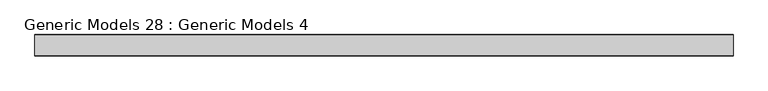
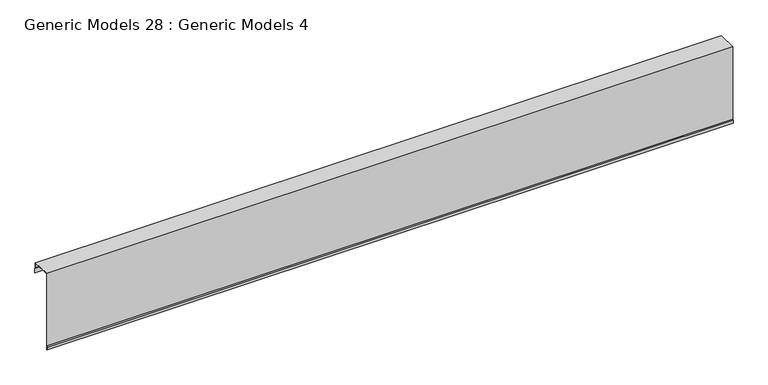
"""IFC4 building model written with IfcOpenShell, lengths in millimetres: proxy geometry, Generic Models 28 : Generic Models 4."""

from ifc_helpers import new_model, si_unit, frame, origin, place, context, project, spatial, polyline, outline, extrude, source, transform, mapped, element, save


def generic_models_28_generic_models_4_6f23a58d(model_context):
    return source(origin(), model_context, "Body", "SweptSolid", [
        extrude(outline(polyline([(-6892.3785185, 127021.0124798), (-6894.9743325, 127028.1444203), (-6894.9743325, 127077.8147702), (-7077.6823532, 127085.4276044), (-7077.6823532, 126394.6532716), (-7079.9703208, 126384.7429952), (-7079.9703208, 126359.7294973), (-7080.7640708, 126359.7294973), (-7080.7640708, 126384.8334316), (-7078.4761032, 126394.743708), (-7078.4761032, 127086.255116), (-6894.1805825, 127078.576136), (-6894.1805825, 127028.2843798), (-6891.5847685, 127021.1524393), (-6891.5847685, 126981.761836), (-6892.3785185, 126981.761836), (-6892.3785185, 127021.0124798)])), frame((2196.9263704, 0.0, 0.0), z_axis=(1.0, 0.0, 0.0), x_axis=(0.0, 1.0, 0.0)), (0.0, 0.0, 1.0), 6189.931498),
    ])


if __name__ == "__main__":
    model = new_model("IFC4")
    model_context = context("Model", 3, world=origin())
    ifc_project = project(units=[si_unit("LENGTHUNIT", "METRE", prefix="MILLI")], contexts=[model_context])
    site = spatial("IfcSite", under=ifc_project)
    building = spatial("IfcBuilding", under=site)
    placement = place(None, origin())
    generic_models_28_generic_models_4_shape = generic_models_28_generic_models_4_6f23a58d(model_context)
    element("IfcBuildingElementProxy", 1, Name="Generic Models 28 : Generic Models 4", ObjectType="Generic Models 28 : Generic Models 4", at=placement, inside=building, context=model_context, shape_type="MappedRepresentation", body=[
        mapped(generic_models_28_generic_models_4_shape, transform((0.0, 0.0, 0.0), x_axis=(1.0, 0.0, 0.0), y_axis=(0.0, 1.0, 0.0), z_axis=(0.0, 0.0, 1.0))),
    ])
    save(model, "model.ifc")

# Revit data of these elements
# Element 1 (IfcBuildingElementProxy, "Generic Models 28 : Generic Models 4")
#   Materials on its faces: "_(2) LAYERS NO. 30 ASTM D226 ASPHALT SATURATED ORGANIC FELT"
# Materials
#   "_(2) LAYERS NO. 30 ASTM D226 ASPHALT SATURATED ORGANIC FELT": class "Generic", colour RGB 67 154 161, transparency 0, Cost = 0
